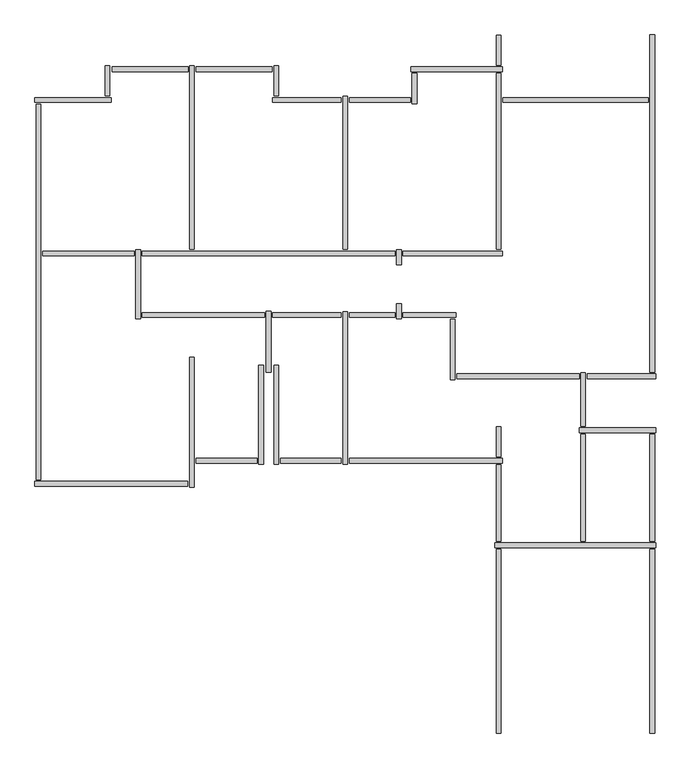
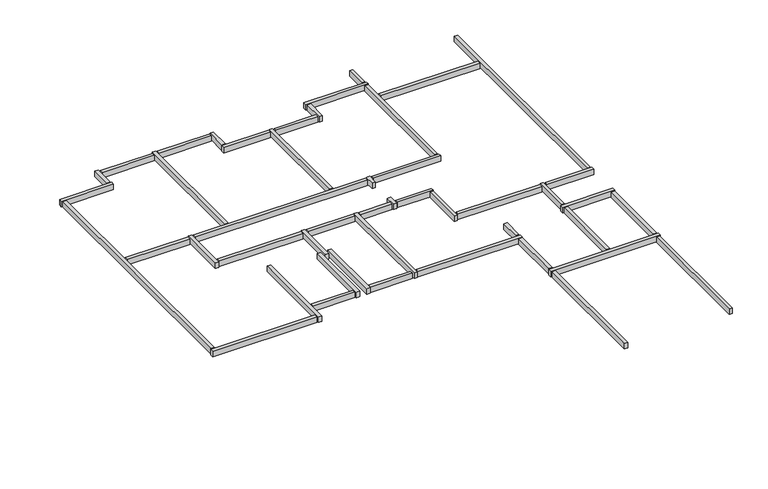
"""IFC4 building model written with IfcOpenShell, lengths in millimetres: beam geometry, Graute viga de respaldo7 : Graute viga de respaldo."""

from ifc_helpers import new_model, si_unit, frame, origin, place, context, project, spatial, polyline, outline, extrude, source, transform, mapped, element, save


def beam_b7f607ab(model_context):
    return source(origin(), model_context, "Body", "SweptSolid", [
        extrude(outline(polyline([(-70718.7587292, 62785.4278788), (-70624.7587292, 62785.4278788), (-70624.7587292, 59195.4278788), (-70718.7587292, 59195.4278788), (-70718.7587292, 62785.4278788)])), frame((0.0, 0.0, 5632.9999999), z_axis=(0.0, 0.0, 1.0), x_axis=(1.0, 0.0, 0.0)), (0.0, 0.0, 1.0), 167.0),
        extrude(outline(polyline([(-67718.7587292, 62785.4278788), (-67624.7587292, 62785.4278788), (-67624.7587292, 59195.4278788), (-67718.7587292, 59195.4278788), (-67718.7587292, 62785.4278788)])), frame((0.0, 0.0, 5632.9999999), z_axis=(0.0, 0.0, 1.0), x_axis=(1.0, 0.0, 0.0)), (0.0, 0.0, 1.0), 167.0),
        extrude(outline(polyline([(-75401.7587292, 64562.4278788), (-75401.7587292, 64468.4278788), (-76591.7587292, 64468.4278788), (-76591.7587292, 64562.4278788), (-75401.7587292, 64562.4278788)])), frame((0.0, 0.0, 5632.9999999), z_axis=(0.0, 0.0, 1.0), x_axis=(1.0, 0.0, 0.0)), (0.0, 0.0, 1.0), 167.0),
        extrude(outline(polyline([(-73751.7587292, 64562.4278788), (-73751.7587292, 64468.4278788), (-74941.7587292, 64468.4278788), (-74941.7587292, 64562.4278788), (-73751.7587292, 64562.4278788)])), frame((0.0, 0.0, 5632.9999999), z_axis=(0.0, 0.0, 1.0), x_axis=(1.0, 0.0, 0.0)), (0.0, 0.0, 1.0), 167.0),
        extrude(outline(polyline([(-77801.7587292, 68612.4278788), (-77801.7587292, 68518.4278788), (-79591.7587292, 68518.4278788), (-79591.7587292, 68612.4278788), (-77801.7587292, 68612.4278788)])), frame((0.0, 0.0, 5632.9999999), z_axis=(0.0, 0.0, 1.0), x_axis=(1.0, 0.0, 0.0)), (0.0, 0.0, 1.0), 167.0),
        extrude(outline(polyline([(-72401.7587292, 71612.4278788), (-72401.7587292, 71518.4278788), (-73591.7587292, 71518.4278788), (-73591.7587292, 71612.4278788), (-72401.7587292, 71612.4278788)])), frame((0.0, 0.0, 5632.9999999), z_axis=(0.0, 0.0, 1.0), x_axis=(1.0, 0.0, 0.0)), (0.0, 0.0, 1.0), 167.0),
        extrude(outline(polyline([(-72274.7587292, 71495.4278788), (-72368.7587292, 71495.4278788), (-72368.7587292, 72085.4278788), (-72274.7587292, 72085.4278788), (-72274.7587292, 71495.4278788)])), frame((0.0, 0.0, 5632.9999999), z_axis=(0.0, 0.0, 1.0), x_axis=(1.0, 0.0, 0.0)), (0.0, 0.0, 1.0), 167.0),
        extrude(outline(polyline([(-70601.7587292, 72212.4278788), (-70601.7587292, 72118.4278788), (-72391.7587292, 72118.4278788), (-72391.7587292, 72212.4278788), (-70601.7587292, 72212.4278788)])), frame((0.0, 0.0, 5632.9999999), z_axis=(0.0, 0.0, 1.0), x_axis=(1.0, 0.0, 0.0)), (0.0, 0.0, 1.0), 167.0),
        extrude(outline(polyline([(-72668.7587292, 68635.4278788), (-72574.7587292, 68635.4278788), (-72574.7587292, 68345.4278788), (-72668.7587292, 68345.4278788), (-72668.7587292, 68635.4278788)])), frame((0.0, 0.0, 5632.9999999), z_axis=(0.0, 0.0, 1.0), x_axis=(1.0, 0.0, 0.0)), (0.0, 0.0, 1.0), 167.0),
        extrude(outline(polyline([(-75251.7587292, 67412.4278788), (-75251.7587292, 67318.4278788), (-77641.7587292, 67318.4278788), (-77641.7587292, 67412.4278788), (-75251.7587292, 67412.4278788)])), frame((0.0, 0.0, 5632.9999999), z_axis=(0.0, 0.0, 1.0), x_axis=(1.0, 0.0, 0.0)), (0.0, 0.0, 1.0), 167.0),
        extrude(outline(polyline([(-73751.7587292, 67412.4278788), (-73751.7587292, 67318.4278788), (-75091.7587292, 67318.4278788), (-75091.7587292, 67412.4278788), (-73751.7587292, 67412.4278788)])), frame((0.0, 0.0, 5632.9999999), z_axis=(0.0, 0.0, 1.0), x_axis=(1.0, 0.0, 0.0)), (0.0, 0.0, 1.0), 167.0),
        extrude(outline(polyline([(-72701.7587292, 67412.4278788), (-72701.7587292, 67318.4278788), (-73591.7587292, 67318.4278788), (-73591.7587292, 67412.4278788), (-72701.7587292, 67412.4278788)])), frame((0.0, 0.0, 5632.9999999), z_axis=(0.0, 0.0, 1.0), x_axis=(1.0, 0.0, 0.0)), (0.0, 0.0, 1.0), 167.0),
        extrude(outline(polyline([(-72668.7587292, 67585.4278788), (-72574.7587292, 67585.4278788), (-72574.7587292, 67295.4278788), (-72668.7587292, 67295.4278788), (-72668.7587292, 67585.4278788)])), frame((0.0, 0.0, 5632.9999999), z_axis=(0.0, 0.0, 1.0), x_axis=(1.0, 0.0, 0.0)), (0.0, 0.0, 1.0), 167.0),
        extrude(outline(polyline([(-71511.7587292, 67412.4278788), (-71511.7587292, 67318.4278788), (-72541.7587292, 67318.4278788), (-72541.7587292, 67412.4278788), (-71511.7587292, 67412.4278788)])), frame((0.0, 0.0, 5632.9999999), z_axis=(0.0, 0.0, 1.0), x_axis=(1.0, 0.0, 0.0)), (0.0, 0.0, 1.0), 167.0),
        extrude(outline(polyline([(-71524.7587292, 66095.4278788), (-71618.7587292, 66095.4278788), (-71618.7587292, 67285.4278788), (-71524.7587292, 67285.4278788), (-71524.7587292, 66095.4278788)])), frame((0.0, 0.0, 5632.9999999), z_axis=(0.0, 0.0, 1.0), x_axis=(1.0, 0.0, 0.0)), (0.0, 0.0, 1.0), 167.0),
        extrude(outline(polyline([(-69091.7587292, 66212.4278788), (-69091.7587292, 66118.4278788), (-71491.7587292, 66118.4278788), (-71491.7587292, 66212.4278788), (-69091.7587292, 66212.4278788)])), frame((0.0, 0.0, 5632.9999999), z_axis=(0.0, 0.0, 1.0), x_axis=(1.0, 0.0, 0.0)), (0.0, 0.0, 1.0), 167.0),
        extrude(outline(polyline([(-73718.7587292, 67430.4278788), (-73624.7587292, 67430.4278788), (-73624.7587292, 64445.4278788), (-73718.7587292, 64445.4278788), (-73718.7587292, 67430.4278788)])), frame((0.0, 0.0, 5632.9999999), z_axis=(0.0, 0.0, 1.0), x_axis=(1.0, 0.0, 0.0)), (0.0, 0.0, 1.0), 167.0),
        extrude(outline(polyline([(-70601.7587292, 64562.4278788), (-70601.7587292, 64468.4278788), (-73591.7587292, 64468.4278788), (-73591.7587292, 64562.4278788), (-70601.7587292, 64562.4278788)])), frame((0.0, 0.0, 5632.9999999), z_axis=(0.0, 0.0, 1.0), x_axis=(1.0, 0.0, 0.0)), (0.0, 0.0, 1.0), 167.0),
        extrude(outline(polyline([(-70718.7587292, 65185.4278788), (-70624.7587292, 65185.4278788), (-70624.7587292, 64595.4278788), (-70718.7587292, 64595.4278788), (-70718.7587292, 65185.4278788)])), frame((0.0, 0.0, 5632.9999999), z_axis=(0.0, 0.0, 1.0), x_axis=(1.0, 0.0, 0.0)), (0.0, 0.0, 1.0), 167.0),
        extrude(outline(polyline([(-70624.7587292, 62945.4278788), (-70718.7587292, 62945.4278788), (-70718.7587292, 64435.4278788), (-70624.7587292, 64435.4278788), (-70624.7587292, 62945.4278788)])), frame((0.0, 0.0, 5632.9999999), z_axis=(0.0, 0.0, 1.0), x_axis=(1.0, 0.0, 0.0)), (0.0, 0.0, 1.0), 167.0),
        extrude(outline(polyline([(-67624.7587292, 62945.4278788), (-67718.7587292, 62945.4278788), (-67718.7587292, 65035.4278788), (-67624.7587292, 65035.4278788), (-67624.7587292, 62945.4278788)])), frame((0.0, 0.0, 5632.9999999), z_axis=(0.0, 0.0, 1.0), x_axis=(1.0, 0.0, 0.0)), (0.0, 0.0, 1.0), 167.0),
        extrude(outline(polyline([(-68974.7587292, 62945.4278788), (-69068.7587292, 62945.4278788), (-69068.7587292, 65035.4278788), (-68974.7587292, 65035.4278788), (-68974.7587292, 62945.4278788)])), frame((0.0, 0.0, 5632.9999999), z_axis=(0.0, 0.0, 1.0), x_axis=(1.0, 0.0, 0.0)), (0.0, 0.0, 1.0), 167.0),
        extrude(outline(polyline([(-69068.7587292, 66235.4278788), (-68974.7587292, 66235.4278788), (-68974.7587292, 65195.4278788), (-69068.7587292, 65195.4278788), (-69068.7587292, 66235.4278788)])), frame((0.0, 0.0, 5632.9999999), z_axis=(0.0, 0.0, 1.0), x_axis=(1.0, 0.0, 0.0)), (0.0, 0.0, 1.0), 167.0),
        extrude(outline(polyline([(-67751.7587292, 71612.4278788), (-67751.7587292, 71518.4278788), (-70591.7587292, 71518.4278788), (-70591.7587292, 71612.4278788), (-67751.7587292, 71612.4278788)])), frame((0.0, 0.0, 5632.9999999), z_axis=(0.0, 0.0, 1.0), x_axis=(1.0, 0.0, 0.0)), (0.0, 0.0, 1.0), 167.0),
        extrude(outline(polyline([(-70624.7587292, 68645.4278788), (-70718.7587292, 68645.4278788), (-70718.7587292, 72085.4278788), (-70624.7587292, 72085.4278788), (-70624.7587292, 68645.4278788)])), frame((0.0, 0.0, 5632.9999999), z_axis=(0.0, 0.0, 1.0), x_axis=(1.0, 0.0, 0.0)), (0.0, 0.0, 1.0), 167.0),
        extrude(outline(polyline([(-70601.7587292, 68612.4278788), (-70601.7587292, 68518.4278788), (-72541.7587292, 68518.4278788), (-72541.7587292, 68612.4278788), (-70601.7587292, 68612.4278788)])), frame((0.0, 0.0, 5632.9999999), z_axis=(0.0, 0.0, 1.0), x_axis=(1.0, 0.0, 0.0)), (0.0, 0.0, 1.0), 167.0),
        extrude(outline(polyline([(-72701.7587292, 68612.4278788), (-72701.7587292, 68518.4278788), (-77641.7587292, 68518.4278788), (-77641.7587292, 68612.4278788), (-72701.7587292, 68612.4278788)])), frame((0.0, 0.0, 5632.9999999), z_axis=(0.0, 0.0, 1.0), x_axis=(1.0, 0.0, 0.0)), (0.0, 0.0, 1.0), 167.0),
        extrude(outline(polyline([(-73718.7587292, 71635.4278788), (-73624.7587292, 71635.4278788), (-73624.7587292, 68645.4278788), (-73718.7587292, 68645.4278788), (-73718.7587292, 71635.4278788)])), frame((0.0, 0.0, 5632.9999999), z_axis=(0.0, 0.0, 1.0), x_axis=(1.0, 0.0, 0.0)), (0.0, 0.0, 1.0), 167.0),
        extrude(outline(polyline([(-75091.7587292, 71518.4278788), (-75091.7587292, 71612.4278788), (-73751.7587292, 71612.4278788), (-73751.7587292, 71518.4278788), (-75091.7587292, 71518.4278788)])), frame((0.0, 0.0, 5632.9999999), z_axis=(0.0, 0.0, 1.0), x_axis=(1.0, 0.0, 0.0)), (0.0, 0.0, 1.0), 167.0),
        extrude(outline(polyline([(-75068.7587292, 72235.4278788), (-74974.7587292, 72235.4278788), (-74974.7587292, 71645.4278788), (-75068.7587292, 71645.4278788), (-75068.7587292, 72235.4278788)])), frame((0.0, 0.0, 5632.9999999), z_axis=(0.0, 0.0, 1.0), x_axis=(1.0, 0.0, 0.0)), (0.0, 0.0, 1.0), 167.0),
        extrude(outline(polyline([(-75101.7587292, 72212.4278788), (-75101.7587292, 72118.4278788), (-76591.7587292, 72118.4278788), (-76591.7587292, 72212.4278788), (-75101.7587292, 72212.4278788)])), frame((0.0, 0.0, 5632.9999999), z_axis=(0.0, 0.0, 1.0), x_axis=(1.0, 0.0, 0.0)), (0.0, 0.0, 1.0), 167.0),
        extrude(outline(polyline([(-78230.736554, 72117.4278788), (-78230.736554, 72212.4278788), (-76741.7587292, 72212.4278788), (-76741.7587292, 72117.4278788), (-78230.736554, 72117.4278788)])), frame((0.0, 0.0, 5617.1856208), z_axis=(0.0, 0.0, 1.0), x_axis=(1.0, 0.0, 0.0)), (0.0, 0.0, 1.0), 165.0),
        extrude(outline(polyline([(-79624.7587292, 64145.4278788), (-79718.7587292, 64145.4278788), (-79718.7587292, 71485.4278788), (-79624.7587292, 71485.4278788), (-79624.7587292, 64145.4278788)])), frame((0.0, 0.0, 5632.9999999), z_axis=(0.0, 0.0, 1.0), x_axis=(1.0, 0.0, 0.0)), (0.0, 0.0, 1.0), 167.0),
        extrude(outline(polyline([(-77674.7587292, 67295.4278788), (-77768.7587292, 67295.4278788), (-77768.7587292, 68640.7810915), (-77674.7587292, 68640.7810915), (-77674.7587292, 67295.4278788)])), frame((0.0, 0.0, 5632.9999999), z_axis=(0.0, 0.0, 1.0), x_axis=(1.0, 0.0, 0.0)), (0.0, 0.0, 1.0), 167.0),
        extrude(outline(polyline([(-75124.7587292, 66245.4278788), (-75218.7587292, 66245.4278788), (-75218.7587292, 67435.4278788), (-75124.7587292, 67435.4278788), (-75124.7587292, 66245.4278788)])), frame((0.0, 0.0, 5632.9999999), z_axis=(0.0, 0.0, 1.0), x_axis=(1.0, 0.0, 0.0)), (0.0, 0.0, 1.0), 167.0),
        extrude(outline(polyline([(-75274.7587292, 64445.4278788), (-75368.7587292, 64445.4278788), (-75368.7587292, 66385.4278788), (-75274.7587292, 66385.4278788), (-75274.7587292, 64445.4278788)])), frame((0.0, 0.0, 5632.9999999), z_axis=(0.0, 0.0, 1.0), x_axis=(1.0, 0.0, 0.0)), (0.0, 0.0, 1.0), 167.0),
        extrude(outline(polyline([(-74974.7587292, 64445.4278788), (-75068.7587292, 64445.4278788), (-75068.7587292, 66385.4278788), (-74974.7587292, 66385.4278788), (-74974.7587292, 64445.4278788)])), frame((0.0, 0.0, 5632.9999999), z_axis=(0.0, 0.0, 1.0), x_axis=(1.0, 0.0, 0.0)), (0.0, 0.0, 1.0), 167.0),
        extrude(outline(polyline([(-76624.7587292, 63995.4278788), (-76718.7587292, 63995.4278788), (-76718.7587292, 66535.4278788), (-76624.7587292, 66535.4278788), (-76624.7587292, 63995.4278788)])), frame((0.0, 0.0, 5632.9999999), z_axis=(0.0, 0.0, 1.0), x_axis=(1.0, 0.0, 0.0)), (0.0, 0.0, 1.0), 167.0),
        extrude(outline(polyline([(-79741.7587292, 64018.4278788), (-79741.7587292, 64112.4278788), (-76751.7587292, 64112.4278788), (-76751.7587292, 64018.4278788), (-79741.7587292, 64018.4278788)])), frame((0.0, 0.0, 5632.9999999), z_axis=(0.0, 0.0, 1.0), x_axis=(1.0, 0.0, 0.0)), (0.0, 0.0, 1.0), 167.0),
        extrude(outline(polyline([(-78368.7587292, 72235.4278788), (-78274.7587292, 72235.4278788), (-78274.7587292, 71645.4278788), (-78368.7587292, 71645.4278788), (-78368.7587292, 72235.4278788)])), frame((0.0, 0.0, 5632.9999999), z_axis=(0.0, 0.0, 1.0), x_axis=(1.0, 0.0, 0.0)), (0.0, 0.0, 1.0), 167.0),
        extrude(outline(polyline([(-78251.7587292, 71612.4278788), (-78251.7587292, 71518.4278788), (-79741.7587292, 71518.4278788), (-79741.7587292, 71612.4278788), (-78251.7587292, 71612.4278788)])), frame((0.0, 0.0, 5632.9999999), z_axis=(0.0, 0.0, 1.0), x_axis=(1.0, 0.0, 0.0)), (0.0, 0.0, 1.0), 167.0),
        extrude(outline(polyline([(-76718.7587292, 72235.4278788), (-76624.7587292, 72235.4278788), (-76624.7587292, 68645.4278788), (-76718.7587292, 68645.4278788), (-76718.7587292, 72235.4278788)])), frame((0.0, 0.0, 5632.9999999), z_axis=(0.0, 0.0, 1.0), x_axis=(1.0, 0.0, 0.0)), (0.0, 0.0, 1.0), 167.0),
        extrude(outline(polyline([(-70718.7587292, 72835.4278788), (-70624.7587292, 72835.4278788), (-70624.7587292, 72245.4278788), (-70718.7587292, 72245.4278788), (-70718.7587292, 72835.4278788)])), frame((0.0, 0.0, 5632.9999999), z_axis=(0.0, 0.0, 1.0), x_axis=(1.0, 0.0, 0.0)), (0.0, 0.0, 1.0), 167.0),
        extrude(outline(polyline([(-67601.7587292, 65162.4278788), (-67601.7587292, 65068.4278788), (-69091.7587292, 65068.4278788), (-69091.7587292, 65162.4278788), (-67601.7587292, 65162.4278788)])), frame((0.0, 0.0, 5632.9999999), z_axis=(0.0, 0.0, 1.0), x_axis=(1.0, 0.0, 0.0)), (0.0, 0.0, 1.0), 167.0),
        extrude(outline(polyline([(-67601.7587292, 62912.4278788), (-67601.7587292, 62818.4278788), (-70741.7587292, 62818.4278788), (-70741.7587292, 62912.4278788), (-67601.7587292, 62912.4278788)])), frame((0.0, 0.0, 5632.9999999), z_axis=(0.0, 0.0, 1.0), x_axis=(1.0, 0.0, 0.0)), (0.0, 0.0, 1.0), 167.0),
        extrude(outline(polyline([(-67601.7587292, 66212.4278788), (-67601.7587292, 66118.4278788), (-68941.7587292, 66118.4278788), (-68941.7587292, 66212.4278788), (-67601.7587292, 66212.4278788)])), frame((0.0, 0.0, 5632.9999999), z_axis=(0.0, 0.0, 1.0), x_axis=(1.0, 0.0, 0.0)), (0.0, 0.0, 1.0), 167.0),
        extrude(outline(polyline([(-67718.7587292, 72837.9577736), (-67624.7587292, 72837.9577736), (-67624.7587292, 66245.4278788), (-67718.7587292, 66245.4278788), (-67718.7587292, 72837.9577736)])), frame((0.0, 0.0, 5632.9999999), z_axis=(0.0, 0.0, 1.0), x_axis=(1.0, 0.0, 0.0)), (0.0, 0.0, 1.0), 167.0),
    ])


if __name__ == "__main__":
    model = new_model("IFC4")
    model_context = context("Model", 3, world=origin())
    ifc_project = project(units=[si_unit("LENGTHUNIT", "METRE", prefix="MILLI")], contexts=[model_context])
    site = spatial("IfcSite", under=ifc_project)
    building = spatial("IfcBuilding", under=site)
    placement = place(None, origin())
    beam_shape = beam_b7f607ab(model_context)
    element("IfcBeam", 1, ObjectType="Graute viga de respaldo7 : Graute viga de respaldo", at=placement, inside=building, context=model_context, shape_type="MappedRepresentation", body=[
        mapped(beam_shape, transform((0.0, 0.0, 0.0), x_axis=(1.0, 0.0, 0.0), y_axis=(0.0, 1.0, 0.0), z_axis=(0.0, 0.0, 1.0))),
    ])
    save(model, "model.ifc")

# Revit data of these elements
# Element 1 (IfcBeam, "Graute viga de respaldo7 : Graute viga de respaldo")
#   Materials on its faces: "Concreto, Faixa de areia/cimento"
# Materials
#   "Concreto, Faixa de areia/cimento": class "Concreto", colour RGB 127 127 127, transparency 0, Description = "Revestimento de laje de concreto", Cost = 0
